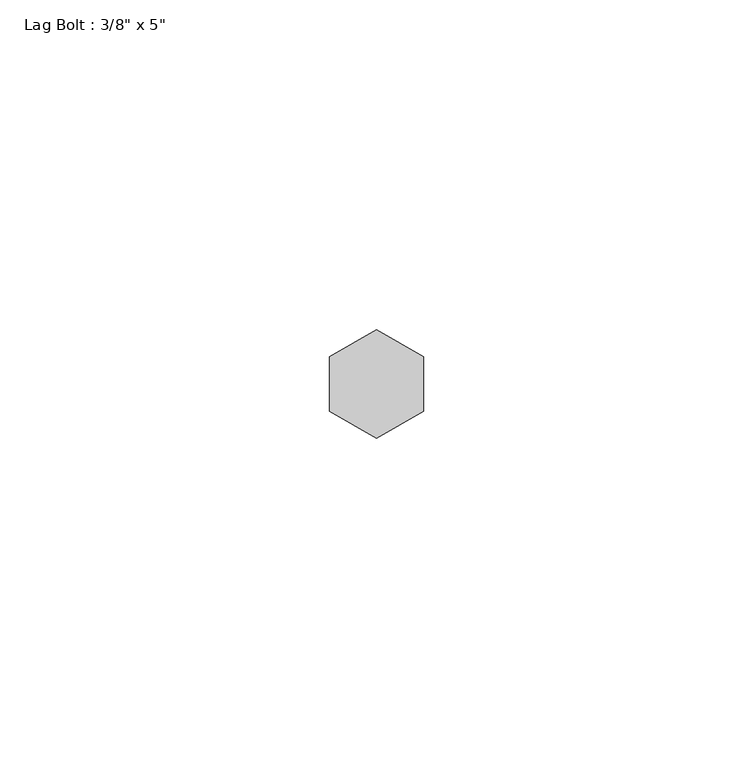
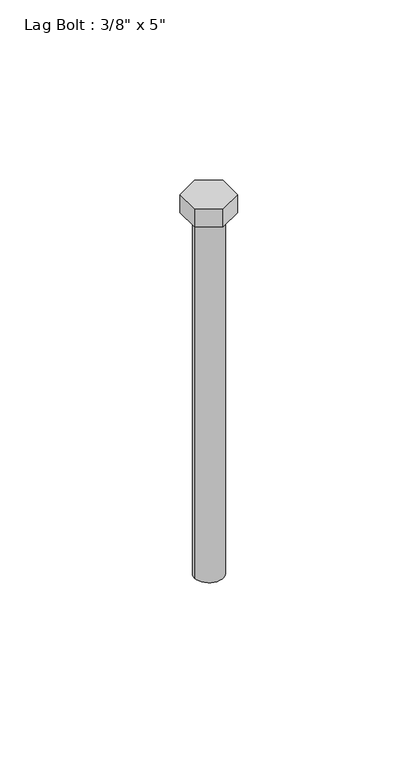
"""IFC4 building model written with IfcOpenShell, lengths in millimetres: proxy geometry."""

from ifc_helpers import new_model, si_unit, point, frame, origin, origin_with_axes, origin_2d, place, context, project, spatial, polyline, circle_curve, trimmed, segment, composite_curve, outline, extrude, source, transform, mapped, element, save


def proxy_c96eb358(model_context):
    return source(origin(), model_context, "Body", "SweptSolid", [
        extrude(outline(polyline([(-7.14375, -4.124446), (-7.14375, 4.124446), (0.0, 8.248892), (7.14375, 4.124446), (7.14375, -4.124446), (0.0, -8.248892), (-7.14375, -4.124446)])), origin_with_axes(), (0.0, 0.0, 1.0), 6.35),
        extrude(outline(composite_curve([segment(trimmed(circle_curve(origin_2d(), 4.7625), [point((-4.7625, 0.0))], [point((4.7625, 0.0))], False, "CARTESIAN"), True, "CONTINUOUS"), segment(trimmed(circle_curve(origin_2d(), 4.7625), [point((4.7625, 0.0))], [point((-4.7625, 0.0))], False, "CARTESIAN"), True, "CONTINUOUS")], self_intersect=False)), frame((0.0, 0.0, -127.0), z_axis=(0.0, 0.0, 1.0), x_axis=(1.0, 0.0, 0.0)), (0.0, 0.0, 1.0), 127.0),
    ])


if __name__ == "__main__":
    model = new_model("IFC4")
    model_context = context("Model", 3, world=origin())
    ifc_project = project(units=[si_unit("LENGTHUNIT", "METRE", prefix="MILLI")], contexts=[model_context])
    site = spatial("IfcSite", under=ifc_project)
    building = spatial("IfcBuilding", under=site)
    placement = place(None, origin())
    proxy_shape = proxy_c96eb358(model_context)
    element("IfcBuildingElementProxy", 1, Name="Lag Bolt : 3/8\" x 5\"", ObjectType="Lag Bolt : 3/8\" x 5\"", at=placement, inside=building, context=model_context, shape_type="MappedRepresentation", body=[
        mapped(proxy_shape, transform((0.0, 0.0, 0.0), x_axis=(1.0, 0.0, 0.0), y_axis=(0.0, 1.0, 0.0), z_axis=(0.0, 0.0, 1.0))),
    ])
    save(model, "model.ifc")

# Revit data of these elements
# Type "Lag Bolt : 3/8\" x 5\""
#   Thickness_of_Substrate [instance default] = 0' - 1"
#   Side = 0' - 0.3252"
#   Radius = 0' - 0 3/16"
#   Length = 0' - 5"
#   Head Size = 0' - 0 9/16"
#   Head Radius = 0' - 0 9/32"
#   Head Height = 0' - 0 1/4"
#   Diameter = 0' - 0 3/8"
#   Default Elevation = 4' - 0"
#   Nut_Visibility [instance default] = no
#   Bolt Material (Size) [instance default] = none
# Element 1 (IfcBuildingElementProxy, "Lag Bolt : 3/8\" x 5\"")
#   Thickness_of_Substrate = 0' - 9 1/4"
#   Bolt Material (Size) = _LAG BOTS - (SEE STRUCT. DWGS)
#   Materials on its faces: "_LAG BOTS - (SEE STRUCT. DWGS)"
# Materials
#   "_LAG BOTS - (SEE STRUCT. DWGS)": class "Metal", colour RGB 199 199 199, transparency 0, Description = "Structural steel 50ksi", Cost = 0
